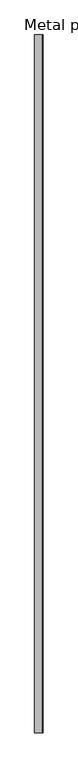
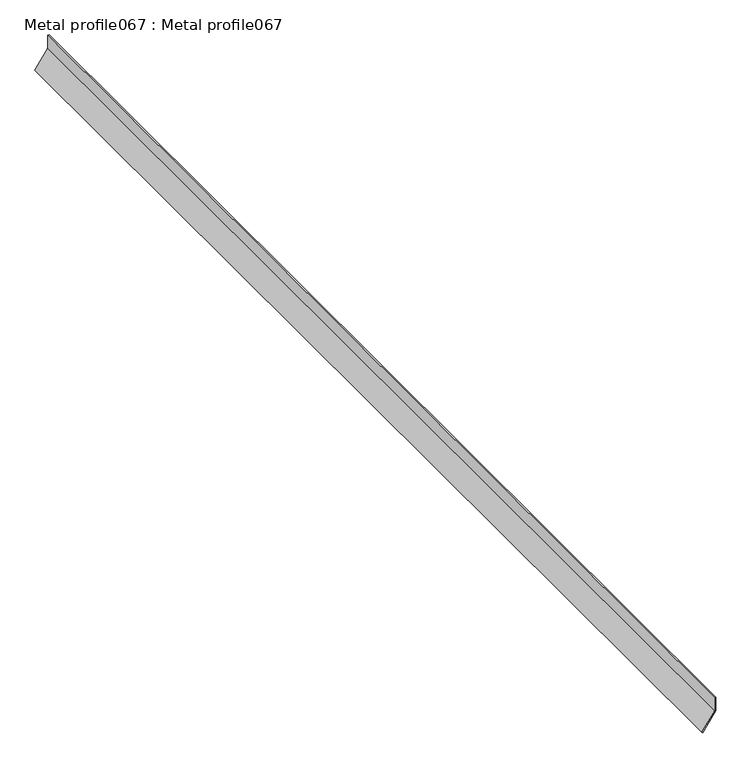
"""IFC4 building model written with IfcOpenShell, lengths in millimetres: proxy geometry, Metal profile067 : Metal profile067."""

from ifc_helpers import new_model, si_unit, frame, origin, place, context, project, spatial, polyline, outline, extrude, source, transform, mapped, element, save


def metal_profile067_metal_profile067_4523fee5(model_context):
    return source(origin(), model_context, "Body", "SweptSolid", [
        extrude(outline(polyline([(43089.9960937, -6495.1103516), (43066.1730094, -6495.1103516), (43034.0291353, -6517.5934749), (43032.8828125, -6515.9545898), (43065.5429687, -6493.1103516), (43089.9960937, -6493.1103516), (43089.9960937, -6495.1103516)])), frame((0.0, 7982.1531721, 0.0), z_axis=(0.0, 1.0, 0.0), x_axis=(0.0, 0.0, 1.0)), (0.0, 0.0, 1.0), 2000.0),
    ])


if __name__ == "__main__":
    model = new_model("IFC4")
    model_context = context("Model", 3, world=origin())
    ifc_project = project(units=[si_unit("LENGTHUNIT", "METRE", prefix="MILLI")], contexts=[model_context])
    site = spatial("IfcSite", under=ifc_project)
    building = spatial("IfcBuilding", under=site)
    placement = place(None, origin())
    metal_profile067_metal_profile067_shape = metal_profile067_metal_profile067_4523fee5(model_context)
    element("IfcBuildingElementProxy", 1, Name="Metal profile067 : Metal profile067", ObjectType="Metal profile067 : Metal profile067", at=placement, inside=building, context=model_context, shape_type="MappedRepresentation", body=[
        mapped(metal_profile067_metal_profile067_shape, transform((0.0, 0.0, 0.0), x_axis=(1.0, 0.0, 0.0), y_axis=(0.0, 1.0, 0.0), z_axis=(0.0, 0.0, 1.0))),
    ])
    save(model, "model.ifc")

# Revit data of these elements
# Type "Metal profile067 : Metal profile067"
#   NameOverride = "Metal profile067"
# Element 1 (IfcBuildingElementProxy, "Metal profile067 : Metal profile067")
#   Materials on its faces: "TRIM CLEAT"
# Materials
#   "TRIM CLEAT": class "Unassigned", colour RGB 255 232 5, transparency 0
